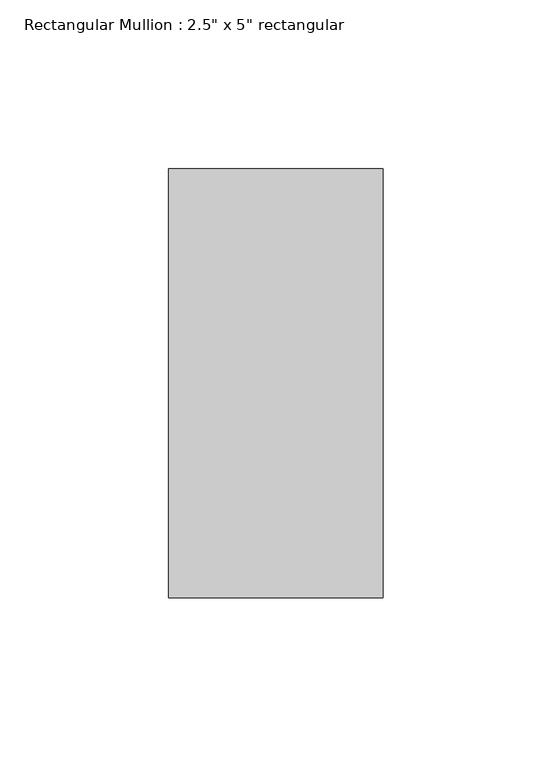
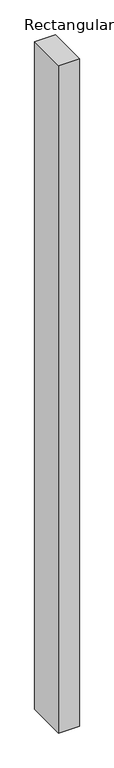
"""IFC4 building model written with IfcOpenShell, lengths in millimetres: member geometry."""

from ifc_helpers import new_model, si_unit, frame, origin, place, context, project, spatial, polyline, outline, extrude, source, transform, mapped, element, save


def member_a50b3cda(model_context):
    return source(origin(), model_context, "Body", "SweptSolid", [
        extrude(outline(polyline([(0.0, 63.5), (0.0, -63.5), (-63.5, -63.5), (-63.5, 63.5), (0.0, 63.5)])), frame((0.0, 0.0, -2165.35), z_axis=(0.0, 0.0, 1.0), x_axis=(1.0, 0.0, 0.0)), (0.0, 0.0, 1.0), 2165.35),
    ])


if __name__ == "__main__":
    model = new_model("IFC4")
    model_context = context("Model", 3, world=origin())
    ifc_project = project(units=[si_unit("LENGTHUNIT", "METRE", prefix="MILLI")], contexts=[model_context])
    site = spatial("IfcSite", under=ifc_project)
    building = spatial("IfcBuilding", under=site)
    placement = place(None, origin())
    member_shape = member_a50b3cda(model_context)
    element("IfcMember", 1, ObjectType="Rectangular Mullion : 2.5\" x 5\" rectangular", at=placement, inside=building, context=model_context, shape_type="MappedRepresentation", body=[
        mapped(member_shape, transform((0.0, 0.0, 0.0), x_axis=(1.0, 0.0, 0.0), y_axis=(0.0, 1.0, 0.0), z_axis=(0.0, 0.0, 1.0))),
    ])
    save(model, "model.ifc")

# Revit data of these elements
# Type "Rectangular Mullion : 2.5\" x 5\" rectangular"
#   built-in parameter 1007304 = 0.416667 (stored number, unit not read)
#   built-in parameter 1007301 = 0.104167 (stored number, unit not read)
#   built-in parameter 1007300 = 0.104167 (stored number, unit not read)
# Element 1 (IfcMember, "Rectangular Mullion : 2.5\" x 5\" rectangular")
#   Materials on its faces: "Metal - Aluminum"
# Materials
#   "Metal - Aluminum": class "Metal", colour RGB 140 140 140, transparency 0
